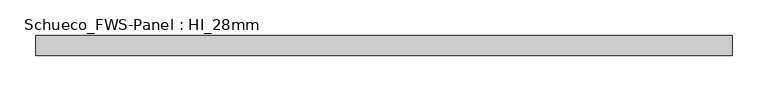
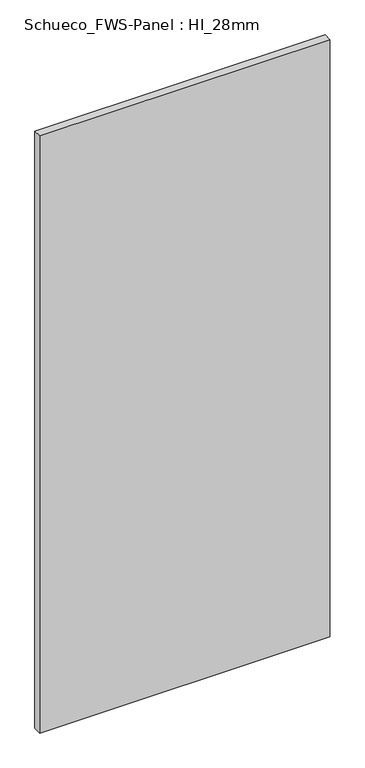
"""IFC4 building model written with IfcOpenShell, lengths in millimetres: plate geometry, Schueco_FWS-Panel : HI_28mm."""

from ifc_helpers import new_model, si_unit, origin, origin_with_axes, place, context, project, spatial, polyline, outline, extrude, source, transform, mapped, element, save


def schueco_fws_panel_hi_28mm_c436cef2(model_context):
    return source(origin(), model_context, "Body", "SweptSolid", [
        extrude(outline(polyline([(-489.0, 0.0), (489.0, 0.0), (489.0, -28.0), (-489.0, -28.0), (-489.0, 0.0)])), origin_with_axes(), (0.0, 0.0, 1.0), 2128.0),
    ])


if __name__ == "__main__":
    model = new_model("IFC4")
    model_context = context("Model", 3, world=origin())
    ifc_project = project(units=[si_unit("LENGTHUNIT", "METRE", prefix="MILLI")], contexts=[model_context])
    site = spatial("IfcSite", under=ifc_project)
    building = spatial("IfcBuilding", under=site)
    placement = place(None, origin())
    schueco_fws_panel_hi_28mm_shape = schueco_fws_panel_hi_28mm_c436cef2(model_context)
    element("IfcPlate", 1, ObjectType="Schueco_FWS-Panel : HI_28mm", at=placement, inside=building, context=model_context, shape_type="MappedRepresentation", body=[
        mapped(schueco_fws_panel_hi_28mm_shape, transform((0.0, 0.0, 0.0), x_axis=(1.0, 0.0, 0.0), y_axis=(0.0, 1.0, 0.0), z_axis=(0.0, 0.0, 1.0))),
    ])
    save(model, "model.ifc")

# Revit data of these elements
# Type "Schueco_FWS-Panel : HI_28mm"
#   Model = "Panel 28mm"
#   Manufacturer = "Schueco International KG"
#   Analytic Construction = "<Keine Auswahl>"
#   Panel thickness = 28 mm
#   Angle right [instance default] = 0.00°
#   Angle left [instance default] = 0.00°
#   AR [instance default] = 0.00°
#   AL [instance default] = 0.00°
#   FWS SI insert unit = no
#   FWS HI insert unit = yes
#   Det_R [instance default] = yes
#   Det_L [instance default] = yes
#   Panel = Alu
# Element 1 (IfcPlate, "Schueco_FWS-Panel : HI_28mm")
#   Materials on its faces: "Alu"
# Materials
#   "Alu": class "Glas", colour RGB 140 140 140, transparency 0
